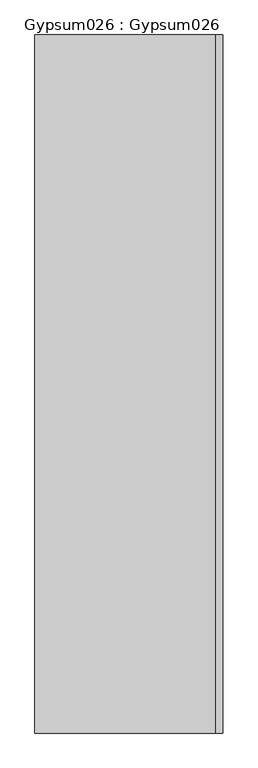
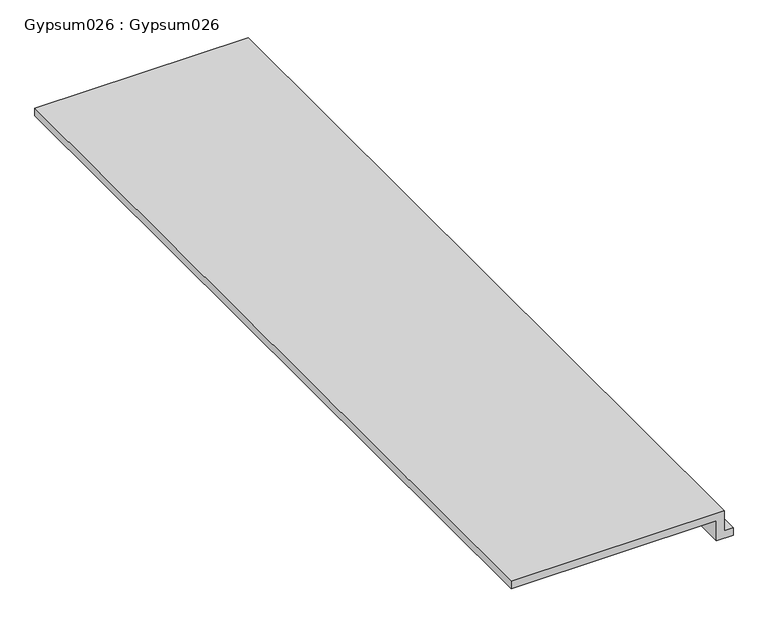
"""IFC4 building model written with IfcOpenShell, lengths in millimetres: proxy geometry, Gypsum026 : Gypsum026."""

from ifc_helpers import new_model, si_unit, frame, origin, place, context, project, spatial, polyline, outline, extrude, source, transform, mapped, element, save


def gypsum026_gypsum026_0701cc7d(model_context):
    return source(origin(), model_context, "Body", "SweptSolid", [
        extrude(outline(polyline([(43005.4089179, 16509.2543635), (43056.2089179, 16509.2543635), (43056.2089179, 15992.0976563), (43037.1589179, 15992.0976563), (43037.1589179, 16490.2043635), (42986.3589179, 16490.2043635), (42986.3589179, 16530.6464844), (43005.4089179, 16530.6464844), (43005.4089179, 16509.2543635)])), frame((0.0, 7982.1435508, 0.0), z_axis=(0.0, 1.0, 0.0), x_axis=(0.0, 0.0, 1.0)), (0.0, 0.0, 1.0), 2000.0),
    ])


if __name__ == "__main__":
    model = new_model("IFC4")
    model_context = context("Model", 3, world=origin())
    ifc_project = project(units=[si_unit("LENGTHUNIT", "METRE", prefix="MILLI")], contexts=[model_context])
    site = spatial("IfcSite", under=ifc_project)
    building = spatial("IfcBuilding", under=site)
    placement = place(None, origin())
    gypsum026_gypsum026_shape = gypsum026_gypsum026_0701cc7d(model_context)
    element("IfcBuildingElementProxy", 1, Name="Gypsum026 : Gypsum026", ObjectType="Gypsum026 : Gypsum026", at=placement, inside=building, context=model_context, shape_type="MappedRepresentation", body=[
        mapped(gypsum026_gypsum026_shape, transform((0.0, 0.0, 0.0), x_axis=(1.0, 0.0, 0.0), y_axis=(0.0, 1.0, 0.0), z_axis=(0.0, 0.0, 1.0))),
    ])
    save(model, "model.ifc")

# Revit data of these elements
# Type "Gypsum026 : Gypsum026"
#   NameOverride = "Gypsum026"
# Element 1 (IfcBuildingElementProxy, "Gypsum026 : Gypsum026")
#   Materials on its faces: "5/8\" GYPSUM BOARD"
# Materials
#   "5/8\" GYPSUM BOARD": class "Unassigned", colour RGB 214 214 214, transparency 0, Cost = 0
